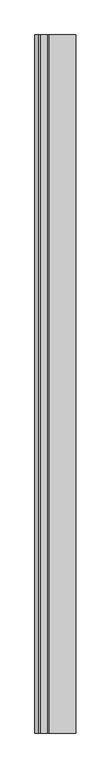
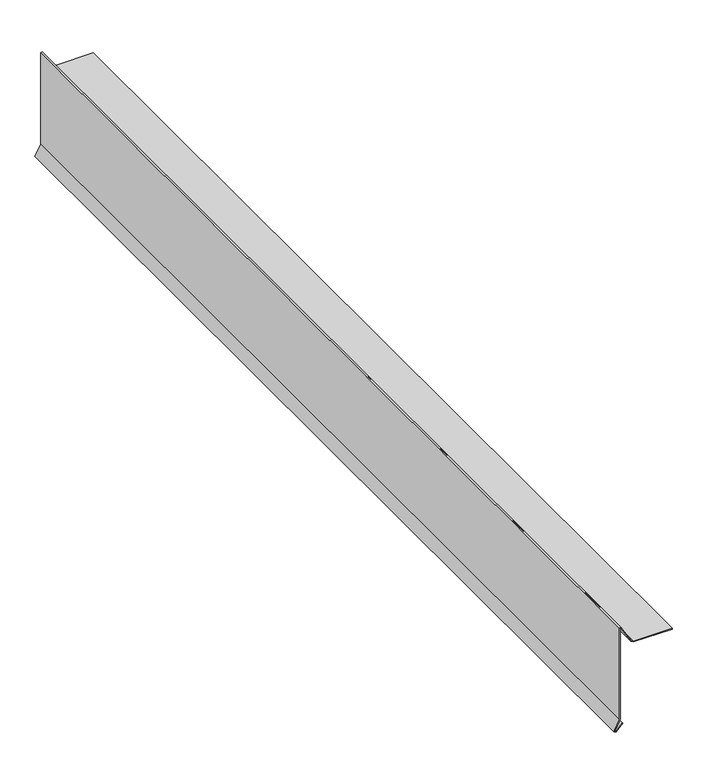
"""IFC4 building model written with IfcOpenShell, lengths in millimetres: proxy geometry, GRAVEL STOP002 3739 : GRAVEL STOP002 3739."""

from ifc_helpers import new_model, si_unit, frame, origin, place, context, project, spatial, polyline, outline, extrude, source, transform, mapped, element, save


def generic_models_e62ea456(model_context):
    return source(origin(), model_context, "Body", "SweptSolid", [
        extrude(outline(polyline([(40077.410403, -5045.5157154), (40091.8049, -5031.1212184), (40092.8027062, -5032.1190245), (40079.2807815, -5045.6409492), (40080.9054201, -5047.7705993), (40101.495749, -5036.5295796), (40293.447969, -5036.5295796), (40293.699878, -5035.5894424), (40258.5078708, -5015.2713276), (40255.9633674, -5010.8641185), (40255.9633674, -4933.0281058), (40257.3744784, -4933.0281058), (40257.3744784, -5010.4860124), (40259.5408757, -5014.2383227), (40295.3431515, -5034.9087762), (40294.5307525, -5037.9406906), (40101.8558531, -5037.9406906), (40080.5182783, -5049.5896595), (40077.410403, -5045.5157154)])), frame((0.0, -1052.8906573, 0.0), z_axis=(0.0, 1.0, 0.0), x_axis=(0.0, 0.0, 1.0)), (0.0, 0.0, 1.0), 2000.25),
    ])


if __name__ == "__main__":
    model = new_model("IFC4")
    model_context = context("Model", 3, world=origin())
    ifc_project = project(units=[si_unit("LENGTHUNIT", "METRE", prefix="MILLI")], contexts=[model_context])
    site = spatial("IfcSite", under=ifc_project)
    building = spatial("IfcBuilding", under=site)
    placement = place(None, origin())
    generic_models_shape = generic_models_e62ea456(model_context)
    element("IfcBuildingElementProxy", 1, Name="GRAVEL STOP002 3739 : GRAVEL STOP002 3739", ObjectType="GRAVEL STOP002 3739 : GRAVEL STOP002 3739", at=placement, inside=building, context=model_context, shape_type="MappedRepresentation", body=[
        mapped(generic_models_shape, transform((0.0, 0.0, 0.0), x_axis=(1.0, 0.0, 0.0), y_axis=(0.0, 1.0, 0.0), z_axis=(0.0, 0.0, 1.0))),
    ])
    save(model, "model.ifc")

# Revit data of these elements
# Type "GRAVEL STOP002 3739 : GRAVEL STOP002 3739"
#   NameOverride = "GRAVEL STOP002"
# Element 1 (IfcBuildingElementProxy, "GRAVEL STOP002 3739 : GRAVEL STOP002 3739")
#   Materials on its faces: "GRAVEL STOP REQUIRED WITH GRAVEL SURFACE SYSTEMS"
# Materials
#   "GRAVEL STOP REQUIRED WITH GRAVEL SURFACE SYSTEMS": class "Unassigned", colour RGB 170 170 127, transparency 0
